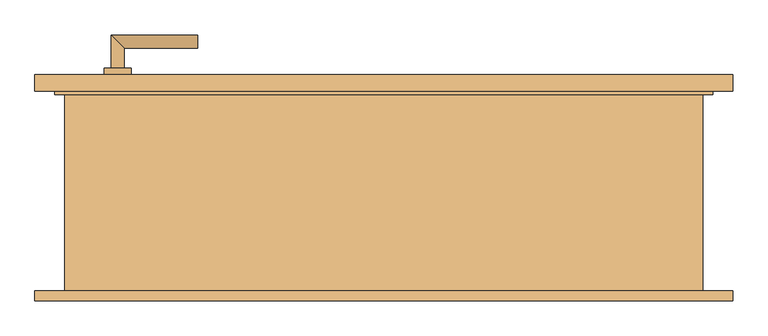
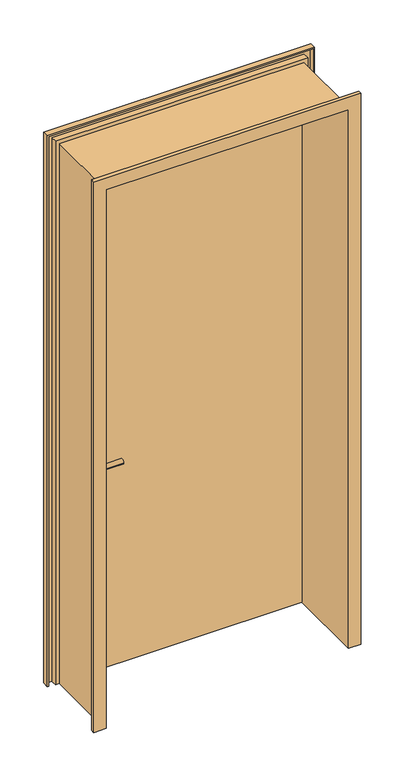
"""IFC4 building model written with IfcOpenShell, lengths in millimetres: door geometry, Drehflügel 1-flg - Variabel : Drehflügel 1-flg - Variabel."""

from ifc_helpers import new_model, si_unit, point, frame, frame_2d, origin, origin_with_axes, place, context, project, spatial, polyline, circle_curve, ellipse_curve, trimmed, segment, composite_curve, outline, extrude, faceted_brep, source, transform, mapped, element, save
from ifc_brep_helpers import plane_surface, cylinder_surface, advanced_brep


def door_334fe5e5(model_context):
    return source(origin(), model_context, "Body", "SolidModel", [
        advanced_brep(
        [(-410.0, 139.4346141, 900.0), (-390.0, 139.4346141, 900.0), (-410.0, 69.4346141, 900.0), (-390.0, 89.4346141, 900.0), (-280.0, 69.4346141, 900.0), (-280.0, 89.4346141, 900.0)],
        [
            (0, 1, circle_curve(frame((-400.0, 139.4346141, 900.0), z_axis=(0.0, 1.0, 0.0), x_axis=(1.0, 0.0, 0.0)), 10.0)),
            (1, 0, circle_curve(frame((-400.0, 139.4346141, 900.0), z_axis=(0.0, 1.0, 0.0), x_axis=(1.0, 0.0, 0.0)), 10.0)),
            (0, 2),
            (2, 3, ellipse_curve(frame((-400.0, 79.4346141, 900.0), z_axis=(-0.7071067811865385, 0.7071067811865565, 0.0), x_axis=(0.7071067811865563, 0.7071067811865386, 0.0)), 14.1421356, 10.0)),
            (3, 1),
            (3, 2, ellipse_curve(frame((-400.0, 79.4346141, 900.0), z_axis=(-0.7071067811865385, 0.7071067811865565, 0.0), x_axis=(0.7071067811865563, 0.7071067811865386, 0.0)), 14.1421356, 10.0)),
            (4, 5, circle_curve(frame((-280.0, 79.4346141, 900.0), z_axis=(1.0, 0.0, 0.0), x_axis=(0.0, 1.0, 0.0)), 10.0)),
            (5, 4, circle_curve(frame((-280.0, 79.4346141, 900.0), z_axis=(1.0, 0.0, 0.0), x_axis=(0.0, 1.0, 0.0)), 10.0)),
            (2, 4),
            (5, 3),
        ],
        [
            plane_surface(frame((-400.0, 139.4346141, -387.7526403), z_axis=(0.0, 1.0, 0.0), x_axis=(0.0, 0.0, 1.0))),
            cylinder_surface(frame((-400.0, 139.4346141, 900.0), z_axis=(0.0, 1.0, 0.0), x_axis=(1.0, 0.0, 0.0)), 10.0),
            plane_surface(frame((-280.0, 79.4346141, -387.7526403), z_axis=(1.0, 0.0, 0.0), x_axis=(0.0, 0.0, 1.0))),
            cylinder_surface(frame((-400.0, 79.4346141, 900.0), z_axis=(-1.0, 0.0, 0.0), x_axis=(0.0, 1.0, 0.0)), 10.0),
        ],
        [
            (0, [[1, 2]]),
            (1, [[-1, 3, 4, 5]]),
            (1, [[-2, -5, 6, -3]]),
            (2, [[7, 8]]),
            (3, [[-4, 9, -8, 10]]),
            (3, [[-6, -10, -7, -9]]),
        ],
    ),
        advanced_brep(
        [(-390.0, 199.4346141, 900.0), (-410.0, 199.4346141, 900.0), (-390.0, 229.4346141, 900.0), (-410.0, 249.4346141, 900.0), (-280.0, 229.4346141, 900.0), (-280.0, 249.4346141, 900.0)],
        [
            (0, 1, circle_curve(frame((-400.0, 199.4346141, 900.0), z_axis=(0.0, -1.0, 0.0), x_axis=(-1.0, 0.0, 0.0)), 10.0)),
            (1, 0, circle_curve(frame((-400.0, 199.4346141, 900.0), z_axis=(0.0, -1.0, 0.0), x_axis=(-1.0, 0.0, 0.0)), 10.0)),
            (0, 2),
            (2, 3, ellipse_curve(frame((-400.0, 239.4346141, 900.0), z_axis=(-0.7071067811865475, -0.7071067811865475, 0.0), x_axis=(0.7071067811865474, -0.7071067811865476, 0.0)), 14.1421356, 10.0)),
            (3, 1),
            (3, 2, ellipse_curve(frame((-400.0, 239.4346141, 900.0), z_axis=(-0.7071067811865475, -0.7071067811865475, 0.0), x_axis=(0.7071067811865474, -0.7071067811865476, 0.0)), 14.1421356, 10.0)),
            (4, 5, circle_curve(frame((-280.0, 239.4346141, 900.0), z_axis=(1.0, 0.0, 0.0), x_axis=(0.0, 1.0, 0.0)), 10.0)),
            (5, 4, circle_curve(frame((-280.0, 239.4346141, 900.0), z_axis=(1.0, 0.0, 0.0), x_axis=(0.0, 1.0, 0.0)), 10.0)),
            (2, 4),
            (5, 3),
        ],
        [
            plane_surface(frame((-400.0, 199.4346141, -387.7526403), z_axis=(0.0, -1.0, 0.0), x_axis=(0.0, 0.0, 1.0))),
            cylinder_surface(frame((-400.0, 199.4346141, 900.0), z_axis=(0.0, -1.0, 0.0), x_axis=(-1.0, 0.0, 0.0)), 10.0),
            plane_surface(frame((-280.0, 239.4346141, -387.7526403), z_axis=(1.0, 0.0, 0.0), x_axis=(0.0, 0.0, 1.0))),
            cylinder_surface(frame((-400.0, 239.4346141, 900.0), z_axis=(-1.0, 0.0, 0.0), x_axis=(0.0, 1.0, 0.0)), 10.0),
        ],
        [
            (0, [[1, 2]]),
            (1, [[-1, 3, 4, 5]]),
            (1, [[-2, -5, 6, -3]]),
            (2, [[7, 8]]),
            (3, [[-4, 9, -8, 10]]),
            (3, [[-6, -10, -7, -9]]),
        ],
    ),
        extrude(outline(composite_curve([segment(trimmed(circle_curve(frame_2d((900.0, -400.0)), 20.0), [point((900.0, -420.0))], [point((900.0, -380.0))], False, "CARTESIAN"), True, "CONTINUOUS"), segment(trimmed(circle_curve(frame_2d((900.0, -400.0)), 20.0), [point((900.0, -380.0))], [point((900.0, -420.0))], False, "CARTESIAN"), True, "CONTINUOUS")], self_intersect=False)), frame((0.0, 129.4346141, 0.0), z_axis=(0.0, 1.0, 0.0), x_axis=(0.0, 0.0, 1.0)), (0.0, 0.0, 1.0), 10.0),
        extrude(outline(composite_curve([segment(trimmed(circle_curve(frame_2d((900.0, -400.0)), 20.0), [point((900.0, -420.0))], [point((900.0, -380.0))], False, "CARTESIAN"), True, "CONTINUOUS"), segment(trimmed(circle_curve(frame_2d((900.0, -400.0)), 20.0), [point((900.0, -380.0))], [point((900.0, -420.0))], False, "CARTESIAN"), True, "CONTINUOUS")], self_intersect=False)), frame((0.0, 189.4346141, 0.0), z_axis=(0.0, 1.0, 0.0), x_axis=(0.0, 0.0, 1.0)), (0.0, 0.0, 1.0), 10.0),
        extrude(outline(polyline([(490.0, 164.4346141), (-490.0, 164.4346141), (-490.0, 189.4346141), (490.0, 189.4346141), (490.0, 164.4346141)])), origin_with_axes(), (0.0, 0.0, 1.0), 2250.0),
        faceted_brep([(524.4603207, -150.5653859, 0.0), (475.0, -150.5653859, 0.0), (475.0, 164.4346141, 0.0), (490.0, 164.4346141, 0.0), (490.0, 189.4346141, 0.0), (524.4603207, 189.4346141, 0.0), (524.4603207, 164.4346141, 0.0), (519.4603207, 164.4346141, 0.0), (519.4603207, 184.4346141, 0.0), (495.0, 184.4346141, 0.0), (495.0, 159.4346141, 0.0), (480.0, 159.4346141, 0.0), (480.0, -145.5653859, 0.0), (519.4603207, -145.5653859, 0.0), (519.4603207, -135.5653859, 0.0), (524.4603207, -135.5653859, 0.0), (524.4603207, -150.5653859, 2284.4603207), (-524.4603207, -150.5653859, 2284.4603207), (-524.4603207, -150.5653859, 0.0), (-475.0, -150.5653859, 0.0), (-475.0, -150.5653859, 2235.0), (475.0, -150.5653859, 2235.0), (475.0, 164.4346141, 2235.0), (-475.0, 164.4346141, 2235.0), (-475.0, 164.4346141, 0.0), (-490.0, 164.4346141, 0.0), (-490.0, 164.4346141, 2250.0), (490.0, 164.4346141, 2250.0), (490.0, 189.4346141, 2250.0), (-490.0, 189.4346141, 2250.0), (-490.0, 189.4346141, 0.0), (-524.4603207, 189.4346141, 0.0), (-524.4603207, 189.4346141, 2284.4603207), (524.4603207, 189.4346141, 2284.4603207), (524.4603207, 164.4346141, 2284.4603207), (-524.4603207, 164.4346141, 2284.4603207), (-524.4603207, 164.4346141, 0.0), (-519.4603207, 164.4346141, 0.0), (-519.4603207, 164.4346141, 2279.4603207), (519.4603207, 164.4346141, 2279.4603207), (519.4603207, 184.4346141, 2279.4603207), (-519.4603207, 184.4346141, 2279.4603207), (-519.4603207, 184.4346141, 0.0), (-495.0, 184.4346141, 0.0), (-495.0, 184.4346141, 2255.0), (495.0, 184.4346141, 2255.0), (495.0, 159.4346141, 2255.0), (-495.0, 159.4346141, 2255.0), (-495.0, 159.4346141, 0.0), (-480.0, 159.4346141, 0.0), (-480.0, 159.4346141, 2240.0), (480.0, 159.4346141, 2240.0), (480.0, -145.5653859, 2240.0), (-480.0, -145.5653859, 2240.0), (-480.0, -145.5653859, 0.0), (-519.4603207, -145.5653859, 0.0), (-519.4603207, -145.5653859, 2279.4603207), (519.4603207, -145.5653859, 2279.4603207), (519.4603207, -135.5653859, 2279.4603207), (-519.4603207, -135.5653859, 2279.4603207), (-519.4603207, -135.5653859, 0.0), (-524.4603207, -135.5653859, 0.0), (-524.4603207, -135.5653859, 2284.4603207), (524.4603207, -135.5653859, 2284.4603207)], [[[0, 1, 2, 3, 4, 5, 6, 7, 8, 9, 10, 11, 12, 13, 14, 15]], [[1, 0, 16, 17, 18, 19, 20, 21]], [[2, 1, 21, 22]], [[3, 2, 22, 23, 24, 25, 26, 27]], [[4, 3, 27, 28]], [[5, 4, 28, 29, 30, 31, 32, 33]], [[6, 5, 33, 34]], [[7, 6, 34, 35, 36, 37, 38, 39]], [[8, 7, 39, 40]], [[9, 8, 40, 41, 42, 43, 44, 45]], [[10, 9, 45, 46]], [[11, 10, 46, 47, 48, 49, 50, 51]], [[12, 11, 51, 52]], [[13, 12, 52, 53, 54, 55, 56, 57]], [[14, 13, 57, 58]], [[15, 14, 58, 59, 60, 61, 62, 63]], [[0, 15, 63, 16]], [[17, 62, 61, 18]], [[18, 61, 60, 55, 54, 49, 48, 43, 42, 37, 36, 31, 30, 25, 24, 19]], [[23, 20, 19, 24]], [[29, 26, 25, 30]], [[35, 32, 31, 36]], [[41, 38, 37, 42]], [[47, 44, 43, 48]], [[53, 50, 49, 54]], [[59, 56, 55, 60]], [[22, 21, 20, 23]], [[28, 27, 26, 29]], [[34, 33, 32, 35]], [[40, 39, 38, 41]], [[46, 45, 44, 47]], [[52, 51, 50, 53]], [[58, 57, 56, 59]], [[16, 63, 62, 17]]]),
    ])


if __name__ == "__main__":
    model = new_model("IFC4")
    model_context = context("Model", 3, world=origin())
    ifc_project = project(units=[si_unit("LENGTHUNIT", "METRE", prefix="MILLI")], contexts=[model_context])
    site = spatial("IfcSite", under=ifc_project)
    building = spatial("IfcBuilding", under=site)
    placement = place(None, origin())
    door_shape = door_334fe5e5(model_context)
    element("IfcDoor", 1, ObjectType="Drehflügel 1-flg - Variabel : Drehflügel 1-flg - Variabel", at=placement, inside=building, context=model_context, shape_type="MappedRepresentation", body=[
        mapped(door_shape, transform((0.0, 0.0, 0.0), x_axis=(1.0, 0.0, 0.0), y_axis=(0.0, 1.0, 0.0), z_axis=(0.0, 0.0, 1.0))),
    ])
    save(model, "model.ifc")

# Revit data of these elements
# Type "Drehflügel 1-flg - Variabel : Drehflügel 1-flg - Variabel"
#   Construction Type Id = "MDOOR"
#   Type Mark = "15"
#   Operation = "SingleSwingRight"
#   Keynote = "16.03"
#   Analytic Construction = "Metall"
#   Thermal Resistance (R) = 0.270117 (m²·K)/W
#   Heat Transfer Coefficient (U) = 3.7021 W/(m²·K)
#   Rough Width [instance default] = 1.000 m
#   Rough Height [instance default] = 2.360 m
#   Höhe Türgriff [instance default] = 0.900 m
#   Height [instance default] = 2.260 m
#   Fußbodenaufbau [instance default] = 0.100 m
#   Width [instance default] = 1.000 m
#   Sichtbarkeit Sturzlinien [instance default] = yes
#   Türgriff auswählen [instance default] = element 217699
#   Türgriff [instance default] = none
#   Türflügel [instance default] = none
#   Rahmen/Pfosten [instance default] = Metall - Lackiert - Grau
#   Visual Light Transmittance = 0
#   Solar Heat Gain Coefficient = 0
#   Function = (empty or 0)
#   Wall Closure = (empty or 0)
# Element 1 (IfcDoor, "Drehflügel 1-flg - Variabel : Drehflügel 1-flg - Variabel")
#   Rough Height = 2.260 m
#   Fußbodenaufbau = 0.000 m
#   Materials on its faces: "Metall - Lackiert - Grau", "Metall - Chrom", "Holz - Birke"
# Materials
#   "Metall - Lackiert - Grau": class "Farbe 1", colour RGB 98 98 98, transparency 0, Cost = 0
#   "Metall - Chrom": class "Metall", colour RGB 247 247 247, transparency 0, Cost = 0
#   "Holz - Birke": class "Holz", colour RGB 213 164 103, transparency 0, Cost = 0
